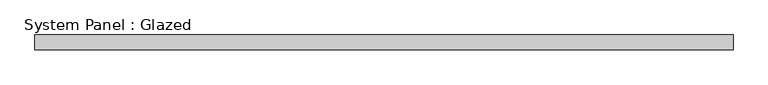
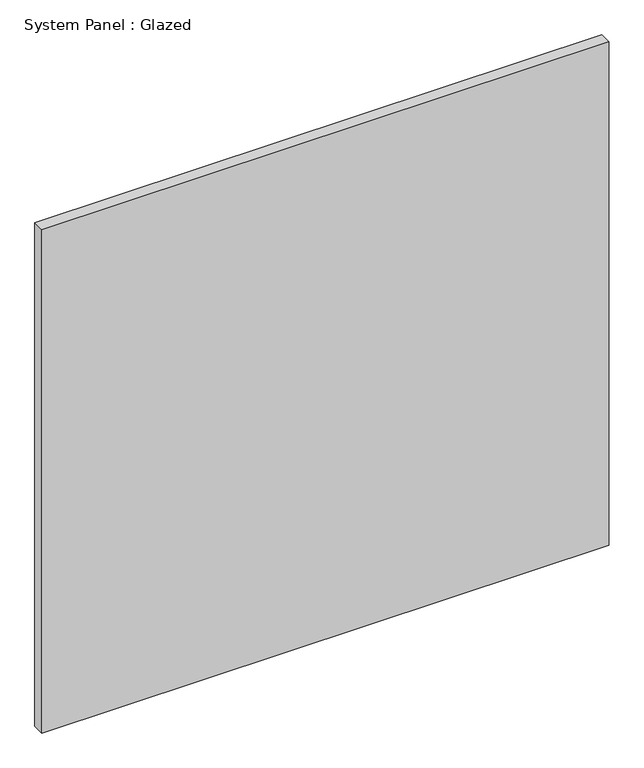
"""IFC4 building model written with IfcOpenShell, lengths in millimetres: plate geometry, System Panel : Glazed."""

import ifcopenshell
import ifcopenshell.guid

model = None  # the IFC model being written
_history = None  # IfcOwnerHistory: only IFC2X3 demands one
_inside = {}  # id of a spatial element -> (the spatial element, [elements in it])
_under = {}  # id of a project, library or spatial element -> (it, [spatial elements below it])
_declared = {}  # id of a project -> (the project, [libraries it declares])
_typed = {}  # id of a type object -> (the type object, [elements of that type])
_made_of = {}  # id of a material, layer set ... -> (it, [elements and type objects made of it])


def new_model(schema):
    """Start an empty IFC model of exactly this schema.

    Asked for "IFC4X3", IfcOpenShell would pick the latest addendum, in which some entities
    have other attributes; the version numbers below select the first issue.
    IFC2X3 requires an IfcOwnerHistory on every rooted entity: one is made here for all.
    """
    global model, _history
    if schema == "IFC4X3":
        model = ifcopenshell.file(schema_version=(4, 3, 0, 0))
    else:
        model = ifcopenshell.file(schema=schema)
    _inside.clear()
    _under.clear()
    _declared.clear()
    _typed.clear()
    _made_of.clear()
    _history = None
    if model.schema == "IFC2X3":
        org = make("IfcOrganization", Name="unknown")
        user = make(
            "IfcPersonAndOrganization",
            ThePerson=make("IfcPerson", FamilyName="unknown"),
            TheOrganization=org,
        )
        app = make(
            "IfcApplication",
            ApplicationDeveloper=org,
            Version="unknown",
            ApplicationFullName="unknown",
            ApplicationIdentifier="unknown",
        )
        _history = make(
            "IfcOwnerHistory",
            OwningUser=user,
            OwningApplication=app,
            ChangeAction="ADDED",
            CreationDate=0,
        )
    return model


def make(cls, **values):
    """One entity of the class cls with the attributes given. An attribute that is None is left unset."""
    return model.create_entity(
        cls, **{name: value for name, value in values.items() if value is not None}
    )


def rooted(cls, **values):
    """An entity with a GlobalId (a new one), such as an element, a storey or a relation."""
    return make(cls, GlobalId=ifcopenshell.guid.new(), OwnerHistory=_history, **values)


def si_unit(unit_type, name, prefix=None):
    """IfcSIUnit, for example si_unit("LENGTHUNIT", "METRE", prefix="MILLI")."""
    return make("IfcSIUnit", UnitType=unit_type, Prefix=prefix, Name=name)


def assignment(units):
    """IfcUnitAssignment: the units of a project."""
    return None if units is None else make("IfcUnitAssignment", Units=units)


def point(xyz):
    """IfcCartesianPoint."""
    return None if xyz is None else make("IfcCartesianPoint", Coordinates=xyz)


def direction(xyz):
    """IfcDirection."""
    return None if xyz is None else make("IfcDirection", DirectionRatios=xyz)


def frame(location, z_axis=None, x_axis=None):
    """IfcAxis2Placement3D, a coordinate frame: its origin and axes. An axis left out is left unset."""
    return make(
        "IfcAxis2Placement3D",
        Location=point(location),
        Axis=direction(z_axis),
        RefDirection=direction(x_axis),
    )


def origin():
    """The frame at (0, 0, 0) with its axes left unset."""
    return frame((0.0, 0.0, 0.0))


def origin_with_axes():
    """The frame at (0, 0, 0) with the z axis (0, 0, 1) and the x axis (1, 0, 0) written out."""
    return frame((0.0, 0.0, 0.0), z_axis=(0.0, 0.0, 1.0), x_axis=(1.0, 0.0, 0.0))


def place(relative_to, where):
    """IfcLocalPlacement: puts the frame where relative to a parent placement (None: the world)."""
    return make(
        "IfcLocalPlacement", PlacementRelTo=relative_to, RelativePlacement=where
    )


def context(
    kind, dimensions, precision=None, world=None, true_north=None, identifier=None
):
    """IfcGeometricRepresentationContext, for example the 3D "Model" context."""
    return make(
        "IfcGeometricRepresentationContext",
        ContextIdentifier=identifier,
        ContextType=kind,
        CoordinateSpaceDimension=dimensions,
        Precision=precision,
        WorldCoordinateSystem=world,
        TrueNorth=true_north,
    )


def project(units=None, contexts=None):
    """IfcProject with its units and contexts."""
    return rooted(
        "IfcProject",
        Name="project",
        RepresentationContexts=contexts,
        UnitsInContext=assignment(units),
    )


def spatial(cls, under=None, at=None, **own):
    """A site, building, storey or space (cls), placed at a placement, below another one or the project."""
    s = rooted(cls, ObjectPlacement=at, **own)
    if under is not None:
        _under.setdefault(under.id(), (under, []))[1].append(s)
    return s


def polyline(points):
    """IfcPolyline through the points."""
    return make("IfcPolyline", Points=[point(p) for p in points])


def outline(outer, holes=None, kind="AREA"):
    """IfcArbitraryClosedProfileDef: a profile drawn as a closed curve; with holes, ...WithVoids."""
    if holes is None:
        return make("IfcArbitraryClosedProfileDef", ProfileType=kind, OuterCurve=outer)
    return make(
        "IfcArbitraryProfileDefWithVoids",
        ProfileType=kind,
        OuterCurve=outer,
        InnerCurves=holes,
    )


def extrude(swept, where, along, depth):
    """IfcExtrudedAreaSolid: the profile swept, set in the frame where, extruded along a direction by depth."""
    return make(
        "IfcExtrudedAreaSolid",
        SweptArea=swept,
        Position=where,
        ExtrudedDirection=direction(along),
        Depth=depth,
    )


def shape(context_of_items, identifier, shape_type, items):
    """IfcShapeRepresentation: the items that make up one representation, for example the "Body"."""
    return make(
        "IfcShapeRepresentation",
        ContextOfItems=context_of_items,
        RepresentationIdentifier=identifier,
        RepresentationType=shape_type,
        Items=items,
    )


def source(mapping_origin, context_of_items, identifier, shape_type, items):
    """IfcRepresentationMap: a shape defined once, which mapped items show again and again."""
    return make(
        "IfcRepresentationMap",
        MappingOrigin=mapping_origin,
        MappedRepresentation=shape(context_of_items, identifier, shape_type, items),
    )


def transform(
    local_origin,
    x_axis=None,
    y_axis=None,
    z_axis=None,
    scale=None,
    scale2=None,
    scale3=None,
    uniform=True,
):
    """IfcCartesianTransformationOperator3D, or its non-uniform kind. x_axis, y_axis, z_axis: its Axis1, 2, 3."""
    if uniform:
        return make(
            "IfcCartesianTransformationOperator3D",
            Axis1=direction(x_axis),
            Axis2=direction(y_axis),
            LocalOrigin=point(local_origin),
            Scale=scale,
            Axis3=direction(z_axis),
        )
    return make(
        "IfcCartesianTransformationOperator3DnonUniform",
        Axis1=direction(x_axis),
        Axis2=direction(y_axis),
        LocalOrigin=point(local_origin),
        Scale=scale,
        Axis3=direction(z_axis),
        Scale2=scale2,
        Scale3=scale3,
    )


def mapped(mapping_source, mapping_target):
    """IfcMappedItem: shows the shape of a source again, moved by a transform."""
    return make(
        "IfcMappedItem", MappingSource=mapping_source, MappingTarget=mapping_target
    )


def made_of(thing, what):
    """Note that an element or type object is made of a material, layer set ...; save() writes the relation."""
    if what is not None:
        _made_of.setdefault(what.id(), (what, []))[1].append(thing)
    return thing


def element(
    cls,
    number,
    at=None,
    inside=None,
    cuts=None,
    type_object=None,
    material=None,
    context=None,
    identifier="Body",
    shape_type=None,
    held_by="IfcProductDefinitionShape",
    body=None,
    shapes=None,
    **own,
):
    """One element of the class cls, such as IfcWall. Its Tag is "e" and its number.

    at: its placement. inside: the storey or other place that contains it. cuts: it is an
    opening in that element (IfcRelVoidsElement). A single representation is given by context,
    identifier, shape_type and body (its items); several are given by shapes. held_by: the class
    of the entity that holds the representations. save() writes the other relations.
    """
    e = rooted(cls, Tag="e%d" % number, ObjectPlacement=at, **own)
    if body is not None:
        shapes = [shape(context, identifier, shape_type, body)]
    if shapes is not None:
        e.Representation = make(held_by, Representations=shapes)
    if inside is not None:
        _inside.setdefault(inside.id(), (inside, []))[1].append(e)
    if cuts is not None:
        rooted(
            "IfcRelVoidsElement", RelatingBuildingElement=cuts, RelatedOpeningElement=e
        )
    if type_object is not None:
        _typed.setdefault(type_object.id(), (type_object, []))[1].append(e)
    return made_of(e, material)


def aggregate(whole, parts):
    """IfcRelAggregates: a whole, such as a stair, and the parts it consists of."""
    return rooted("IfcRelAggregates", RelatingObject=whole, RelatedObjects=parts)


def save(model, path):
    """Write the relations noted so far, then the file.

    IfcRelAggregates (storeys below a building ...), IfcRelContainedInSpatialStructure (elements
    in a storey), IfcRelDefinesByType, IfcRelAssociatesMaterial and IfcRelDeclares: one each for
    every whole, place, type object, material and project.
    """
    for whole, parts in _under.values():
        aggregate(whole, parts)
    for where, things in _inside.values():
        rooted(
            "IfcRelContainedInSpatialStructure",
            RelatedElements=things,
            RelatingStructure=where,
        )
    for kind, things in _typed.values():
        rooted("IfcRelDefinesByType", RelatedObjects=things, RelatingType=kind)
    for what, things in _made_of.values():
        rooted("IfcRelAssociatesMaterial", RelatedObjects=things, RelatingMaterial=what)
    for by, libraries in _declared.values():
        rooted("IfcRelDeclares", RelatingContext=by, RelatedDefinitions=libraries)
    model.write(path)


def system_panel_glazed_dc26df31(model_context):
    return source(origin(), model_context, "Body", "SweptSolid", [
        extrude(outline(polyline([(599.0166667, 19.05), (-599.0166667, 19.05), (-599.0166667, 44.45), (599.0166667, 44.45), (599.0166667, 19.05)])), origin_with_axes(), (0.0, 0.0, 1.0), 1123.95),
    ])


if __name__ == "__main__":
    model = new_model("IFC4")
    model_context = context("Model", 3, world=origin())
    ifc_project = project(units=[si_unit("LENGTHUNIT", "METRE", prefix="MILLI")], contexts=[model_context])
    site = spatial("IfcSite", under=ifc_project)
    building = spatial("IfcBuilding", under=site)
    placement = place(None, origin())
    system_panel_glazed_shape = system_panel_glazed_dc26df31(model_context)
    element("IfcPlate", 1, ObjectType="System Panel : Glazed", at=placement, inside=building, context=model_context, shape_type="MappedRepresentation", body=[
        mapped(system_panel_glazed_shape, transform((0.0, 0.0, 0.0), x_axis=(1.0, 0.0, 0.0), y_axis=(0.0, 1.0, 0.0), z_axis=(0.0, 0.0, 1.0))),
    ])
    save(model, "model.ifc")

# Revit data of these elements
# Element 1 (IfcPlate, "System Panel : Glazed")
#   Materials on its faces: "Glass"
# Materials
#   "Glass": class "Glass", colour RGB 218 227 224, transparency 0.85, Description = "Soda Lime Glass", Cost = 0
